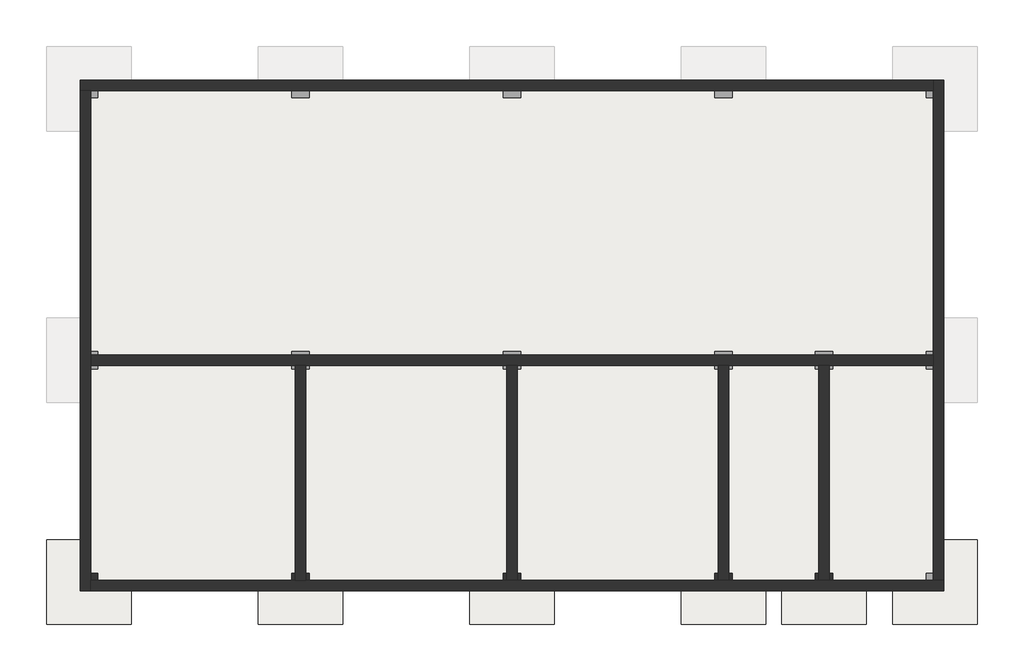
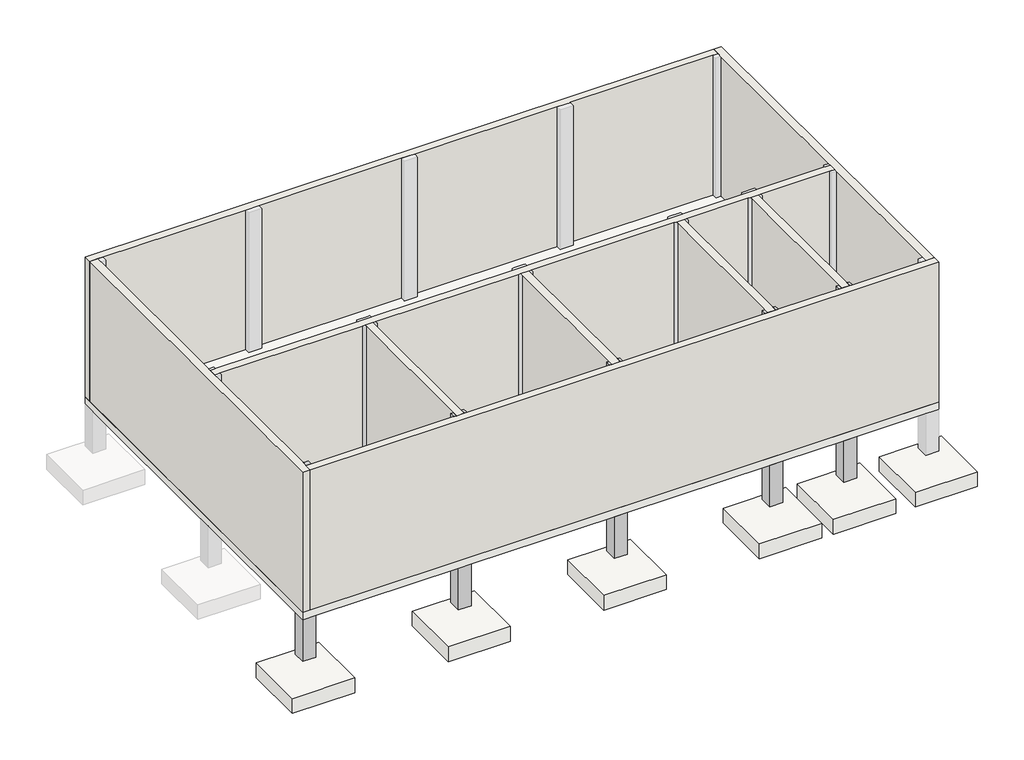
# One storey, part 1 of 2: 10 columns, 9 walls, 7 slabs.
"""IFC4 building model written with IfcOpenShell, lengths in millimetres."""

import ifcopenshell
import ifcopenshell.guid

model = None  # the IFC model being written
_history = None  # IfcOwnerHistory: only IFC2X3 demands one
_inside = {}  # id of a spatial element -> (the spatial element, [elements in it])
_under = {}  # id of a project, library or spatial element -> (it, [spatial elements below it])
_declared = {}  # id of a project -> (the project, [libraries it declares])
_typed = {}  # id of a type object -> (the type object, [elements of that type])
_made_of = {}  # id of a material, layer set ... -> (it, [elements and type objects made of it])


def new_model(schema):
    """Start an empty IFC model of exactly this schema.

    Asked for "IFC4X3", IfcOpenShell would pick the latest addendum, in which some entities
    have other attributes; the version numbers below select the first issue.
    IFC2X3 requires an IfcOwnerHistory on every rooted entity: one is made here for all.
    """
    global model, _history
    if schema == "IFC4X3":
        model = ifcopenshell.file(schema_version=(4, 3, 0, 0))
    else:
        model = ifcopenshell.file(schema=schema)
    _inside.clear()
    _under.clear()
    _declared.clear()
    _typed.clear()
    _made_of.clear()
    _history = None
    if model.schema == "IFC2X3":
        org = make("IfcOrganization", Name="unknown")
        user = make(
            "IfcPersonAndOrganization",
            ThePerson=make("IfcPerson", FamilyName="unknown"),
            TheOrganization=org,
        )
        app = make(
            "IfcApplication",
            ApplicationDeveloper=org,
            Version="unknown",
            ApplicationFullName="unknown",
            ApplicationIdentifier="unknown",
        )
        _history = make(
            "IfcOwnerHistory",
            OwningUser=user,
            OwningApplication=app,
            ChangeAction="ADDED",
            CreationDate=0,
        )
    return model


def make(cls, **values):
    """One entity of the class cls with the attributes given. An attribute that is None is left unset."""
    return model.create_entity(
        cls, **{name: value for name, value in values.items() if value is not None}
    )


def rooted(cls, **values):
    """An entity with a GlobalId (a new one), such as an element, a storey or a relation."""
    return make(cls, GlobalId=ifcopenshell.guid.new(), OwnerHistory=_history, **values)


def si_unit(unit_type, name, prefix=None):
    """IfcSIUnit, for example si_unit("LENGTHUNIT", "METRE", prefix="MILLI")."""
    return make("IfcSIUnit", UnitType=unit_type, Prefix=prefix, Name=name)


def assignment(units):
    """IfcUnitAssignment: the units of a project."""
    return None if units is None else make("IfcUnitAssignment", Units=units)


def point(xyz):
    """IfcCartesianPoint."""
    return None if xyz is None else make("IfcCartesianPoint", Coordinates=xyz)


def direction(xyz):
    """IfcDirection."""
    return None if xyz is None else make("IfcDirection", DirectionRatios=xyz)


def frame(location, z_axis=None, x_axis=None):
    """IfcAxis2Placement3D, a coordinate frame: its origin and axes. An axis left out is left unset."""
    return make(
        "IfcAxis2Placement3D",
        Location=point(location),
        Axis=direction(z_axis),
        RefDirection=direction(x_axis),
    )


def origin():
    """The frame at (0, 0, 0) with its axes left unset."""
    return frame((0.0, 0.0, 0.0))


def place(relative_to, where):
    """IfcLocalPlacement: puts the frame where relative to a parent placement (None: the world)."""
    return make(
        "IfcLocalPlacement", PlacementRelTo=relative_to, RelativePlacement=where
    )


def context(
    kind, dimensions, precision=None, world=None, true_north=None, identifier=None
):
    """IfcGeometricRepresentationContext, for example the 3D "Model" context."""
    return make(
        "IfcGeometricRepresentationContext",
        ContextIdentifier=identifier,
        ContextType=kind,
        CoordinateSpaceDimension=dimensions,
        Precision=precision,
        WorldCoordinateSystem=world,
        TrueNorth=true_north,
    )


def project(units=None, contexts=None):
    """IfcProject with its units and contexts."""
    return rooted(
        "IfcProject",
        Name="project",
        RepresentationContexts=contexts,
        UnitsInContext=assignment(units),
    )


def spatial(cls, under=None, at=None, **own):
    """A site, building, storey or space (cls), placed at a placement, below another one or the project."""
    s = rooted(cls, ObjectPlacement=at, **own)
    if under is not None:
        _under.setdefault(under.id(), (under, []))[1].append(s)
    return s


def polyline(points):
    """IfcPolyline through the points."""
    return make("IfcPolyline", Points=[point(p) for p in points])


def outline(outer, holes=None, kind="AREA"):
    """IfcArbitraryClosedProfileDef: a profile drawn as a closed curve; with holes, ...WithVoids."""
    if holes is None:
        return make("IfcArbitraryClosedProfileDef", ProfileType=kind, OuterCurve=outer)
    return make(
        "IfcArbitraryProfileDefWithVoids",
        ProfileType=kind,
        OuterCurve=outer,
        InnerCurves=holes,
    )


def extrude(swept, where, along, depth):
    """IfcExtrudedAreaSolid: the profile swept, set in the frame where, extruded along a direction by depth."""
    return make(
        "IfcExtrudedAreaSolid",
        SweptArea=swept,
        Position=where,
        ExtrudedDirection=direction(along),
        Depth=depth,
    )


def faces_of(points, faces, orient=None, outer=None):
    """IfcFace entities. A face is a list of loops; a loop is a list of indices into points, from 0.

    orient and outer hold one flag for each loop. By default every Orientation is true, the
    first loop of a face is its IfcFaceOuterBound and the others are IfcFaceBound.
    """
    made = []
    for i, loops in enumerate(faces):
        bounds = []
        for j, loop in enumerate(loops):
            is_outer = j == 0 if outer is None else outer[i][j]
            bounds.append(
                make(
                    "IfcFaceOuterBound" if is_outer else "IfcFaceBound",
                    Bound=make("IfcPolyLoop", Polygon=[points[k] for k in loop]),
                    Orientation=True if orient is None else orient[i][j],
                )
            )
        made.append(make("IfcFace", Bounds=bounds))
    return made


def faceted_brep(points, faces, orient=None, outer=None, voids=None):
    """IfcFacetedBrep: a solid bounded by flat faces; with voids (closed shells), ...WithVoids."""
    shared = [point(p) for p in points]
    hull = make("IfcClosedShell", CfsFaces=faces_of(shared, faces, orient, outer))
    if voids is None:
        return make("IfcFacetedBrep", Outer=hull)
    return make(
        "IfcFacetedBrepWithVoids",
        Outer=hull,
        Voids=[
            make(cls, CfsFaces=faces_of(shared, fs, o, b)) for cls, fs, o, b in voids
        ],
    )


def shape(context_of_items, identifier, shape_type, items):
    """IfcShapeRepresentation: the items that make up one representation, for example the "Body"."""
    return make(
        "IfcShapeRepresentation",
        ContextOfItems=context_of_items,
        RepresentationIdentifier=identifier,
        RepresentationType=shape_type,
        Items=items,
    )


def source(mapping_origin, context_of_items, identifier, shape_type, items):
    """IfcRepresentationMap: a shape defined once, which mapped items show again and again."""
    return make(
        "IfcRepresentationMap",
        MappingOrigin=mapping_origin,
        MappedRepresentation=shape(context_of_items, identifier, shape_type, items),
    )


def transform(
    local_origin,
    x_axis=None,
    y_axis=None,
    z_axis=None,
    scale=None,
    scale2=None,
    scale3=None,
    uniform=True,
):
    """IfcCartesianTransformationOperator3D, or its non-uniform kind. x_axis, y_axis, z_axis: its Axis1, 2, 3."""
    if uniform:
        return make(
            "IfcCartesianTransformationOperator3D",
            Axis1=direction(x_axis),
            Axis2=direction(y_axis),
            LocalOrigin=point(local_origin),
            Scale=scale,
            Axis3=direction(z_axis),
        )
    return make(
        "IfcCartesianTransformationOperator3DnonUniform",
        Axis1=direction(x_axis),
        Axis2=direction(y_axis),
        LocalOrigin=point(local_origin),
        Scale=scale,
        Axis3=direction(z_axis),
        Scale2=scale2,
        Scale3=scale3,
    )


def mapped(mapping_source, mapping_target):
    """IfcMappedItem: shows the shape of a source again, moved by a transform."""
    return make(
        "IfcMappedItem", MappingSource=mapping_source, MappingTarget=mapping_target
    )


def made_of(thing, what):
    """Note that an element or type object is made of a material, layer set ...; save() writes the relation."""
    if what is not None:
        _made_of.setdefault(what.id(), (what, []))[1].append(thing)
    return thing


def element(
    cls,
    number,
    at=None,
    inside=None,
    cuts=None,
    type_object=None,
    material=None,
    context=None,
    identifier="Body",
    shape_type=None,
    held_by="IfcProductDefinitionShape",
    body=None,
    shapes=None,
    **own,
):
    """One element of the class cls, such as IfcWall. Its Tag is "e" and its number.

    at: its placement. inside: the storey or other place that contains it. cuts: it is an
    opening in that element (IfcRelVoidsElement). A single representation is given by context,
    identifier, shape_type and body (its items); several are given by shapes. held_by: the class
    of the entity that holds the representations. save() writes the other relations.
    """
    e = rooted(cls, Tag="e%d" % number, ObjectPlacement=at, **own)
    if body is not None:
        shapes = [shape(context, identifier, shape_type, body)]
    if shapes is not None:
        e.Representation = make(held_by, Representations=shapes)
    if inside is not None:
        _inside.setdefault(inside.id(), (inside, []))[1].append(e)
    if cuts is not None:
        rooted(
            "IfcRelVoidsElement", RelatingBuildingElement=cuts, RelatedOpeningElement=e
        )
    if type_object is not None:
        _typed.setdefault(type_object.id(), (type_object, []))[1].append(e)
    return made_of(e, material)


def aggregate(whole, parts):
    """IfcRelAggregates: a whole, such as a stair, and the parts it consists of."""
    return rooted("IfcRelAggregates", RelatingObject=whole, RelatedObjects=parts)


def save(model, path):
    """Write the relations noted so far, then the file.

    IfcRelAggregates (storeys below a building ...), IfcRelContainedInSpatialStructure (elements
    in a storey), IfcRelDefinesByType, IfcRelAssociatesMaterial and IfcRelDeclares: one each for
    every whole, place, type object, material and project.
    """
    for whole, parts in _under.values():
        aggregate(whole, parts)
    for where, things in _inside.values():
        rooted(
            "IfcRelContainedInSpatialStructure",
            RelatedElements=things,
            RelatingStructure=where,
        )
    for kind, things in _typed.values():
        rooted("IfcRelDefinesByType", RelatedObjects=things, RelatingType=kind)
    for what, things in _made_of.values():
        rooted("IfcRelAssociatesMaterial", RelatedObjects=things, RelatingMaterial=what)
    for by, libraries in _declared.values():
        rooted("IfcRelDeclares", RelatingContext=by, RelatedDefinitions=libraries)
    model.write(path)


def foundation_rectangular_non_pile_2400_x_2400_x_600mm_9fdc1d6b(model_context):
    return source(origin(), model_context, "Body", "SweptSolid", [
        extrude(outline(polyline([(1200.0, 1200.0), (1200.0, -1200.0), (-1200.0, -1200.0), (-1200.0, 1200.0), (1200.0, 1200.0)])), frame((0.0, 0.0, -600.0), z_axis=(0.0, 0.0, 1.0), x_axis=(1.0, 0.0, 0.0)), (0.0, 0.0, 1.0), 600.0),
    ])


model = new_model("IFC4")

# Units and contexts
model_context = context("Model", 3, world=origin())
ifc_project = project(units=[si_unit("LENGTHUNIT", "METRE", prefix="MILLI")], contexts=[model_context])

# Site, building, storey
site = spatial("IfcSite", under=ifc_project)
building = spatial("IfcBuilding", under=site)
storey = spatial("IfcBuildingStorey", under=building, Name="1st FL GL+200", Elevation=0.0)

# Columns
placement = place(None, origin())
element("IfcColumn", 1, ObjectType="RC_Column_Rectangular : 500 x 500mm", at=placement, inside=storey, context=model_context, shape_type="SweptSolid", body=[
    extrude(outline(polyline([(-18445.7273237, -4314.0236875), (-18445.7273237, -4814.0236875), (-18945.7273237, -4814.0236875), (-18945.7273237, -4314.0236875), (-18445.7273237, -4314.0236875)])), frame((0.0, 0.0, -2000.0), z_axis=(0.0, 0.0, 1.0), x_axis=(1.0, 0.0, 0.0)), (0.0, 0.0, 1.0), 1700.0),
])
element("IfcColumn", 2, ObjectType="RC_Column_Rectangular : 500 x 500mm", at=placement, inside=storey, context=model_context, shape_type="SweptSolid", body=[
    extrude(outline(polyline([(-12445.7273237, -4314.0236875), (-12445.7273237, -4814.0236875), (-12945.7273237, -4814.0236875), (-12945.7273237, -4314.0236875), (-12445.7273237, -4314.0236875)])), frame((0.0, 0.0, -2000.0), z_axis=(0.0, 0.0, 1.0), x_axis=(1.0, 0.0, 0.0)), (0.0, 0.0, 1.0), 1700.0),
])
element("IfcColumn", 3, ObjectType="RC_Column_Rectangular : 500 x 500mm", at=placement, inside=storey, context=model_context, shape_type="SweptSolid", body=[
    extrude(outline(polyline([(-6445.7273237, -4314.0236875), (-6445.7273237, -4814.0236875), (-6945.7273237, -4814.0236875), (-6945.7273237, -4314.0236875), (-6445.7273237, -4314.0236875)])), frame((0.0, 0.0, -2000.0), z_axis=(0.0, 0.0, 1.0), x_axis=(1.0, 0.0, 0.0)), (0.0, 0.0, 1.0), 1700.0),
])
element("IfcColumn", 4, ObjectType="RC_Column_Rectangular : 500 x 500mm", at=placement, inside=storey, context=model_context, shape_type="SweptSolid", body=[
    extrude(outline(polyline([(-445.7273237, -4314.0236875), (-445.7273237, -4814.0236875), (-945.7273237, -4814.0236875), (-945.7273237, -4314.0236875), (-445.7273237, -4314.0236875)])), frame((0.0, 0.0, -2000.0), z_axis=(0.0, 0.0, 1.0), x_axis=(1.0, 0.0, 0.0)), (0.0, 0.0, 1.0), 1700.0),
])
element("IfcColumn", 5, ObjectType="RC_Column_Rectangular : 500 x 500mm", at=placement, inside=storey, context=model_context, shape_type="SweptSolid", body=[
    extrude(outline(polyline([(2404.2726763, -4314.0236875), (2404.2726763, -4814.0236875), (1904.2726763, -4814.0236875), (1904.2726763, -4314.0236875), (2404.2726763, -4314.0236875)])), frame((0.0, 0.0, -2000.0), z_axis=(0.0, 0.0, 1.0), x_axis=(1.0, 0.0, 0.0)), (0.0, 0.0, 1.0), 1700.0),
])
element("IfcColumn", 6, ObjectType="RC_Column_Rectangular : 500 x 500mm", at=placement, inside=storey, context=model_context, shape_type="Brep", body=[
    faceted_brep([(-18645.7273237, -4314.0236875, 0.0), (-18445.7273237, -4314.0236875, 0.0), (-18445.7273237, -4514.0236875, 0.0), (-18645.7273237, -4514.0236875, 0.0), (-18445.7273237, -4314.0236875, 5700.0), (-18645.7273237, -4314.0236875, 5300.0), (-18645.7273237, -4314.0236875, 5700.0), (-18595.7273237, -4314.0236875, 5700.0), (-18445.7273237, -4514.0236875, 5700.0), (-18645.7273237, -4514.0236875, 5700.0)], [[[0, 1, 2, 3]], [[4, 1, 0, 5, 6, 7]], [[1, 4, 8, 2]], [[4, 7, 6, 9, 8]], [[6, 5, 0, 3, 9]], [[3, 2, 8, 9]]]),
])
element("IfcColumn", 7, ObjectType="RC_Column_Rectangular : 500 x 500mm", at=placement, inside=storey, context=model_context, shape_type="Brep", body=[
    faceted_brep([(-12945.7273237, -4514.0236875, 0.0), (-12945.7273237, -4314.0236875, 0.0), (-12845.7273237, -4314.0236875, 0.0), (-12845.7273237, -4514.0236875, 0.0), (-12945.7273237, -4314.0236875, 5700.0), (-12945.7273237, -4514.0236875, 5300.0), (-12945.7273237, -4514.0236875, 5700.0), (-12945.7273237, -4464.0236875, 5700.0), (-12845.7273237, -4314.0236875, 5300.0), (-12845.7273237, -4314.0236875, 5700.0), (-12845.7273237, -4514.0236875, 5700.0), (-12870.7273237, -4314.0236875, 5700.0)], [[[0, 1, 2, 3]], [[4, 1, 0, 5, 6, 7]], [[3, 2, 8, 9, 10]], [[1, 4, 11, 9, 8, 2]], [[4, 7, 6, 10, 9, 11]], [[6, 5, 0, 3, 10]]]),
    faceted_brep([(-12445.7273237, -4314.0236875, 5700.0), (-12445.7273237, -4314.0236875, 0.0), (-12545.7273237, -4314.0236875, 0.0), (-12545.7273237, -4314.0236875, 5300.0), (-12545.7273237, -4314.0236875, 5700.0), (-12520.7273237, -4314.0236875, 5700.0), (-12445.7273237, -4464.0236875, 5700.0), (-12445.7273237, -4514.0236875, 5700.0), (-12445.7273237, -4514.0236875, 5300.0), (-12445.7273237, -4514.0236875, 0.0), (-12545.7273237, -4514.0236875, 5700.0), (-12545.7273237, -4514.0236875, 0.0)], [[[0, 1, 2, 3, 4, 5]], [[1, 0, 6, 7, 8, 9]], [[7, 6, 0, 5, 4, 10]], [[9, 8, 7, 10, 11]], [[2, 11, 10, 4, 3]], [[1, 9, 11, 2]]]),
])
element("IfcColumn", 8, ObjectType="RC_Column_Rectangular : 500 x 500mm", at=placement, inside=storey, context=model_context, shape_type="Brep", body=[
    faceted_brep([(-6945.7273237, -4514.0236875, 0.0), (-6945.7273237, -4314.0236875, 0.0), (-6845.7273237, -4314.0236875, 0.0), (-6845.7273237, -4514.0236875, 0.0), (-6945.7273237, -4314.0236875, 5700.0), (-6945.7273237, -4514.0236875, 5300.0), (-6945.7273237, -4514.0236875, 5700.0), (-6945.7273237, -4464.0236875, 5700.0), (-6845.7273237, -4314.0236875, 5300.0), (-6845.7273237, -4314.0236875, 5700.0), (-6845.7273237, -4514.0236875, 5700.0), (-6870.7273237, -4314.0236875, 5700.0)], [[[0, 1, 2, 3]], [[4, 1, 0, 5, 6, 7]], [[3, 2, 8, 9, 10]], [[1, 4, 11, 9, 8, 2]], [[4, 7, 6, 10, 9, 11]], [[6, 5, 0, 3, 10]]]),
    faceted_brep([(-6445.7273237, -4314.0236875, 5700.0), (-6445.7273237, -4314.0236875, 0.0), (-6545.7273237, -4314.0236875, 0.0), (-6545.7273237, -4314.0236875, 5300.0), (-6545.7273237, -4314.0236875, 5700.0), (-6520.7273237, -4314.0236875, 5700.0), (-6445.7273237, -4464.0236875, 5700.0), (-6445.7273237, -4514.0236875, 5700.0), (-6445.7273237, -4514.0236875, 5300.0), (-6445.7273237, -4514.0236875, 0.0), (-6545.7273237, -4514.0236875, 5700.0), (-6545.7273237, -4514.0236875, 0.0)], [[[0, 1, 2, 3, 4, 5]], [[1, 0, 6, 7, 8, 9]], [[7, 6, 0, 5, 4, 10]], [[9, 8, 7, 10, 11]], [[2, 11, 10, 4, 3]], [[1, 9, 11, 2]]]),
])
element("IfcColumn", 9, ObjectType="RC_Column_Rectangular : 500 x 500mm", at=placement, inside=storey, context=model_context, shape_type="Brep", body=[
    faceted_brep([(-945.7273237, -4514.0236875, 0.0), (-945.7273237, -4314.0236875, 0.0), (-845.7273237, -4314.0236875, 0.0), (-845.7273237, -4514.0236875, 0.0), (-945.7273237, -4314.0236875, 5700.0), (-945.7273237, -4514.0236875, 5300.0), (-945.7273237, -4514.0236875, 5700.0), (-945.7273237, -4464.0236875, 5700.0), (-845.7273237, -4314.0236875, 5300.0), (-845.7273237, -4314.0236875, 5700.0), (-845.7273237, -4514.0236875, 5700.0), (-870.7273237, -4314.0236875, 5700.0)], [[[0, 1, 2, 3]], [[4, 1, 0, 5, 6, 7]], [[3, 2, 8, 9, 10]], [[1, 4, 11, 9, 8, 2]], [[4, 7, 6, 10, 9, 11]], [[6, 5, 0, 3, 10]]]),
    faceted_brep([(-445.7273237, -4314.0236875, 5700.0), (-445.7273237, -4314.0236875, 0.0), (-545.7273237, -4314.0236875, 0.0), (-545.7273237, -4314.0236875, 5300.0), (-545.7273237, -4314.0236875, 5700.0), (-520.7273237, -4314.0236875, 5700.0), (-445.7273237, -4464.0236875, 5700.0), (-445.7273237, -4514.0236875, 5700.0), (-445.7273237, -4514.0236875, 5300.0), (-445.7273237, -4514.0236875, 0.0), (-545.7273237, -4514.0236875, 5700.0), (-545.7273237, -4514.0236875, 0.0)], [[[0, 1, 2, 3, 4, 5]], [[1, 0, 6, 7, 8, 9]], [[7, 6, 0, 5, 4, 10]], [[9, 8, 7, 10, 11]], [[2, 11, 10, 4, 3]], [[1, 9, 11, 2]]]),
])
element("IfcColumn", 10, ObjectType="RC_Column_Rectangular : 500 x 500mm", at=placement, inside=storey, context=model_context, shape_type="Brep", body=[
    faceted_brep([(1904.2726763, -4514.0236875, 0.0), (1904.2726763, -4314.0236875, 0.0), (2004.2726763, -4314.0236875, 0.0), (2004.2726763, -4514.0236875, 0.0), (1904.2726763, -4314.0236875, 5700.0), (1904.2726763, -4514.0236875, 5300.0), (1904.2726763, -4514.0236875, 5700.0), (1904.2726763, -4464.0236875, 5700.0), (2004.2726763, -4314.0236875, 5300.0), (2004.2726763, -4314.0236875, 5700.0), (2004.2726763, -4514.0236875, 5700.0), (1979.2726763, -4314.0236875, 5700.0)], [[[0, 1, 2, 3]], [[4, 1, 0, 5, 6, 7]], [[3, 2, 8, 9, 10]], [[1, 4, 11, 9, 8, 2]], [[4, 7, 6, 10, 9, 11]], [[6, 5, 0, 3, 10]]]),
    faceted_brep([(2404.2726763, -4314.0236875, 5700.0), (2404.2726763, -4314.0236875, 0.0), (2304.2726763, -4314.0236875, 0.0), (2304.2726763, -4314.0236875, 5300.0), (2304.2726763, -4314.0236875, 5700.0), (2329.2726763, -4314.0236875, 5700.0), (2404.2726763, -4464.0236875, 5700.0), (2404.2726763, -4514.0236875, 5700.0), (2404.2726763, -4514.0236875, 5300.0), (2404.2726763, -4514.0236875, 0.0), (2304.2726763, -4514.0236875, 5700.0), (2304.2726763, -4514.0236875, 0.0)], [[[0, 1, 2, 3, 4, 5]], [[1, 0, 6, 7, 8, 9]], [[7, 6, 0, 5, 4, 10]], [[9, 8, 7, 10, 11]], [[2, 11, 10, 4, 3]], [[1, 9, 11, 2]]]),
])

# Slabs
element("IfcSlab", 11, ObjectType="H_FL_ACS_RC Slab_T150", at=placement, inside=storey, context=model_context, shape_type="Brep", body=[
    faceted_brep([(5554.2726763, -4814.0236875, -300.0), (5054.2726763, -4814.0236875, -300.0), (2404.2726763, -4814.0236875, -300.0), (1904.2726763, -4814.0236875, -300.0), (-445.7273237, -4814.0236875, -300.0), (-945.7273237, -4814.0236875, -300.0), (-6445.7273237, -4814.0236875, -300.0), (-6945.7273237, -4814.0236875, -300.0), (-12445.7273237, -4814.0236875, -300.0), (-12945.7273237, -4814.0236875, -300.0), (-18445.7273237, -4814.0236875, -300.0), (-18945.7273237, -4814.0236875, -300.0), (-18945.7273237, -4314.0236875, -300.0), (-18945.7273237, 1485.9763125, -300.0), (-18945.7273237, 1985.9763125, -300.0), (-18945.7273237, 9185.9763125, -300.0), (-18945.7273237, 9685.9763125, -300.0), (-18445.7273237, 9685.9763125, -300.0), (-12945.7273237, 9685.9763125, -300.0), (-12445.7273237, 9685.9763125, -300.0), (-6945.7273237, 9685.9763125, -300.0), (-6445.7273237, 9685.9763125, -300.0), (-945.7273237, 9685.9763125, -300.0), (-445.7273237, 9685.9763125, -300.0), (5054.2726763, 9685.9763125, -300.0), (5554.2726763, 9685.9763125, -300.0), (5554.2726763, 9185.9763125, -300.0), (5554.2726763, 1985.9763125, -300.0), (5554.2726763, 1485.9763125, -300.0), (5554.2726763, -4314.0236875, -300.0), (5554.2726763, -4814.0236875, 0.0), (5554.2726763, 9685.9763125, 0.0), (-18945.7273237, 9685.9763125, 0.0), (-18945.7273237, -4814.0236875, 0.0)], [[[0, 1, 2, 3, 4, 5, 6, 7, 8, 9, 10, 11, 12, 13, 14, 15, 16, 17, 18, 19, 20, 21, 22, 23, 24, 25, 26, 27, 28, 29]], [[30, 31, 32, 33]], [[11, 10, 9, 8, 7, 6, 5, 4, 3, 2, 1, 0, 30, 33]], [[16, 15, 14, 13, 12, 11, 33, 32]], [[25, 24, 23, 22, 21, 20, 19, 18, 17, 16, 32, 31]], [[0, 29, 28, 27, 26, 25, 31, 30]]]),
])
foundation_rectangular_non_pile_2400_x_2400_x_600mm_shape = foundation_rectangular_non_pile_2400_x_2400_x_600mm_9fdc1d6b(model_context)
element("IfcSlab", 12, ObjectType="Foundation Rectangular(Non-Pile) : 2400 x 2400 x 600mm", at=placement, inside=storey, context=model_context, shape_type="MappedRepresentation", body=[
    mapped(foundation_rectangular_non_pile_2400_x_2400_x_600mm_shape, transform((-18695.7273237, -4564.0236875, -2600.0), x_axis=(1.0, 0.0, 0.0), y_axis=(0.0, 1.0, 0.0), z_axis=(0.0, 0.0, 1.0))),
])
element("IfcSlab", 13, ObjectType="Foundation Rectangular(Non-Pile) : 2400 x 2400 x 600mm", at=placement, inside=storey, context=model_context, shape_type="MappedRepresentation", body=[
    mapped(foundation_rectangular_non_pile_2400_x_2400_x_600mm_shape, transform((-12695.7273237, -4564.0236875, -2600.0), x_axis=(1.0, 0.0, 0.0), y_axis=(0.0, 1.0, 0.0), z_axis=(0.0, 0.0, 1.0))),
])
element("IfcSlab", 14, ObjectType="Foundation Rectangular(Non-Pile) : 2400 x 2400 x 600mm", at=placement, inside=storey, context=model_context, shape_type="MappedRepresentation", body=[
    mapped(foundation_rectangular_non_pile_2400_x_2400_x_600mm_shape, transform((-6695.7273237, -4564.0236875, -2600.0), x_axis=(1.0, 0.0, 0.0), y_axis=(0.0, 1.0, 0.0), z_axis=(0.0, 0.0, 1.0))),
])
element("IfcSlab", 15, ObjectType="Foundation Rectangular(Non-Pile) : 2400 x 2400 x 600mm", at=placement, inside=storey, context=model_context, shape_type="MappedRepresentation", body=[
    mapped(foundation_rectangular_non_pile_2400_x_2400_x_600mm_shape, transform((-695.7273237, -4564.0236875, -2600.0), x_axis=(1.0, 0.0, 0.0), y_axis=(0.0, 1.0, 0.0), z_axis=(0.0, 0.0, 1.0))),
])
element("IfcSlab", 16, ObjectType="Foundation Rectangular(Non-Pile) : 2400 x 2400 x 600mm", at=placement, inside=storey, context=model_context, shape_type="MappedRepresentation", body=[
    mapped(foundation_rectangular_non_pile_2400_x_2400_x_600mm_shape, transform((5304.2726763, -4564.0236875, -2600.0), x_axis=(1.0, 0.0, 0.0), y_axis=(0.0, 1.0, 0.0), z_axis=(0.0, 0.0, 1.0))),
])
element("IfcSlab", 17, ObjectType="Foundation Rectangular(Non-Pile) : 2400 x 2400 x 600mm", at=placement, inside=storey, context=model_context, shape_type="MappedRepresentation", body=[
    mapped(foundation_rectangular_non_pile_2400_x_2400_x_600mm_shape, transform((2154.2726763, -4564.0236875, -2600.0), x_axis=(1.0, 0.0, 0.0), y_axis=(0.0, 1.0, 0.0), z_axis=(0.0, 0.0, 1.0))),
])

# Walls
element("IfcWall", 18, ObjectType="일반 - 300mm", at=placement, inside=storey, context=model_context, shape_type="Brep", body=[
    faceted_brep([(-18945.7273237, 9385.9763125, 0.0), (-18645.7273237, 9385.9763125, 0.0), (-18445.7273237, 9385.9763125, 0.0), (-12945.7273237, 9385.9763125, 0.0), (-12445.7273237, 9385.9763125, 0.0), (-6945.7273237, 9385.9763125, 0.0), (-6445.7273237, 9385.9763125, 0.0), (-945.7273237, 9385.9763125, 0.0), (-445.7273237, 9385.9763125, 0.0), (5054.2726763, 9385.9763125, 0.0), (5254.2726763, 9385.9763125, 0.0), (5254.2726763, 9385.9763125, 5300.0), (5254.2726763, 9385.9763125, 5700.0), (5054.2726763, 9385.9763125, 5700.0), (-433.0273237, 9385.9763125, 5700.0), (-445.7273237, 9385.9763125, 5700.0), (-945.7273237, 9385.9763125, 5700.0), (-6445.7273237, 9385.9763125, 5700.0), (-6945.7273237, 9385.9763125, 5700.0), (-12445.7273237, 9385.9763125, 5700.0), (-12945.7273237, 9385.9763125, 5700.0), (-18445.7273237, 9385.9763125, 5700.0), (-18645.7273237, 9385.9763125, 5700.0), (-18945.7273237, 9385.9763125, 5700.0), (5254.2726763, 9685.9763125, 0.0), (-18945.7273237, 9685.9763125, 0.0), (-18945.7273237, 9685.9763125, 5700.0), (5254.2726763, 9685.9763125, 5700.0)], [[[0, 1, 2, 3, 4, 5, 6, 7, 8, 9, 10, 11, 12, 13, 14, 15, 16, 17, 18, 19, 20, 21, 22, 23]], [[24, 25, 26, 27]], [[10, 9, 8, 7, 6, 5, 4, 3, 2, 1, 0, 25, 24]], [[25, 0, 23, 26]], [[10, 24, 27, 12, 11]], [[23, 22, 21, 20, 19, 18, 17, 16, 15, 14, 13, 12, 27, 26]]]),
])
element("IfcWall", 19, ObjectType="일반 - 300mm", at=placement, inside=storey, context=model_context, shape_type="Brep", body=[
    faceted_brep([(-18645.7273237, -4814.0236875, 0.0), (-18645.7273237, -4514.0236875, 0.0), (-18645.7273237, -4314.0236875, 0.0), (-18645.7273237, 1485.9763125, 0.0), (-18645.7273237, 1585.9763125, 0.0), (-18645.7273237, 1885.9763125, 0.0), (-18645.7273237, 1985.9763125, 0.0), (-18645.7273237, 9185.9763125, 0.0), (-18645.7273237, 9385.9763125, 0.0), (-18645.7273237, 9385.9763125, 5700.0), (-18645.7273237, 9185.9763125, 5700.0), (-18645.7273237, 1985.9763125, 5700.0), (-18645.7273237, 1885.9763125, 5700.0), (-18645.7273237, 1585.9763125, 5700.0), (-18645.7273237, 1485.9763125, 5700.0), (-18645.7273237, -4314.0236875, 5700.0), (-18645.7273237, -4514.0236875, 5700.0), (-18645.7273237, -4814.0236875, 5700.0), (-18945.7273237, 9385.9763125, 0.0), (-18945.7273237, -4814.0236875, 0.0), (-18945.7273237, -4814.0236875, 5700.0), (-18945.7273237, 9385.9763125, 5700.0)], [[[0, 1, 2, 3, 4, 5, 6, 7, 8, 9, 10, 11, 12, 13, 14, 15, 16, 17]], [[18, 19, 20, 21]], [[8, 7, 6, 5, 4, 3, 2, 1, 0, 19, 18]], [[19, 0, 17, 20]], [[8, 18, 21, 9]], [[17, 16, 15, 14, 13, 12, 11, 10, 9, 21, 20]]]),
])
element("IfcWall", 20, ObjectType="일반 - 300mm", at=placement, inside=storey, context=model_context, shape_type="Brep", body=[
    faceted_brep([(5554.2726763, -4514.0236875, 0.0), (5254.2726763, -4514.0236875, 0.0), (5054.2726763, -4514.0236875, 0.0), (2404.2726763, -4514.0236875, 0.0), (2304.2726763, -4514.0236875, 0.0), (2004.2726763, -4514.0236875, 0.0), (1904.2726763, -4514.0236875, 0.0), (-445.7273237, -4514.0236875, 0.0), (-545.7273237, -4514.0236875, 0.0), (-845.7273237, -4514.0236875, 0.0), (-945.7273237, -4514.0236875, 0.0), (-6445.7273237, -4514.0236875, 0.0), (-6545.7273237, -4514.0236875, 0.0), (-6845.7273237, -4514.0236875, 0.0), (-6945.7273237, -4514.0236875, 0.0), (-12445.7273237, -4514.0236875, 0.0), (-12545.7273237, -4514.0236875, 0.0), (-12845.7273237, -4514.0236875, 0.0), (-12945.7273237, -4514.0236875, 0.0), (-18445.7273237, -4514.0236875, 0.0), (-18645.7273237, -4514.0236875, 0.0), (-18645.7273237, -4514.0236875, 5300.0), (-18645.7273237, -4514.0236875, 5700.0), (-18445.7273237, -4514.0236875, 5700.0), (-12945.7273237, -4514.0236875, 5700.0), (-12845.7273237, -4514.0236875, 5700.0), (-12545.7273237, -4514.0236875, 5700.0), (-12445.7273237, -4514.0236875, 5700.0), (-6945.7273237, -4514.0236875, 5700.0), (-6845.7273237, -4514.0236875, 5700.0), (-6545.7273237, -4514.0236875, 5700.0), (-6445.7273237, -4514.0236875, 5700.0), (-945.7273237, -4514.0236875, 5700.0), (-845.7273237, -4514.0236875, 5700.0), (-545.7273237, -4514.0236875, 5700.0), (-445.7273237, -4514.0236875, 5700.0), (1904.2726763, -4514.0236875, 5700.0), (2004.2726763, -4514.0236875, 5700.0), (2304.2726763, -4514.0236875, 5700.0), (2404.2726763, -4514.0236875, 5700.0), (5054.2726763, -4514.0236875, 5700.0), (5254.2726763, -4514.0236875, 5700.0), (5554.2726763, -4514.0236875, 5700.0), (-18645.7273237, -4814.0236875, 0.0), (5554.2726763, -4814.0236875, 0.0), (5554.2726763, -4814.0236875, 5700.0), (-18645.7273237, -4814.0236875, 5700.0)], [[[0, 1, 2, 3, 4, 5, 6, 7, 8, 9, 10, 11, 12, 13, 14, 15, 16, 17, 18, 19, 20, 21, 22, 23, 24, 25, 26, 27, 28, 29, 30, 31, 32, 33, 34, 35, 36, 37, 38, 39, 40, 41, 42]], [[43, 44, 45, 46]], [[20, 19, 18, 17, 16, 15, 14, 13, 12, 11, 10, 9, 8, 7, 6, 5, 4, 3, 2, 1, 0, 44, 43]], [[44, 0, 42, 45]], [[20, 43, 46, 22, 21]], [[42, 41, 40, 39, 38, 37, 36, 35, 34, 33, 32, 31, 30, 29, 28, 27, 26, 25, 24, 23, 22, 46, 45]]]),
])
element("IfcWall", 21, ObjectType="일반 - 300mm", at=placement, inside=storey, context=model_context, shape_type="Brep", body=[
    faceted_brep([(5254.2726763, 9685.9763125, 0.0), (5254.2726763, 9385.9763125, 0.0), (5254.2726763, 9185.9763125, 0.0), (5254.2726763, 1985.9763125, 0.0), (5254.2726763, 1885.9763125, 0.0), (5254.2726763, 1585.9763125, 0.0), (5254.2726763, 1485.9763125, 0.0), (5254.2726763, -4314.0236875, 0.0), (5254.2726763, -4514.0236875, 0.0), (5254.2726763, -4514.0236875, 5700.0), (5254.2726763, -4314.0236875, 5700.0), (5254.2726763, 1485.9763125, 5700.0), (5254.2726763, 1585.9763125, 5700.0), (5254.2726763, 1885.9763125, 5700.0), (5254.2726763, 1985.9763125, 5700.0), (5254.2726763, 9185.9763125, 5700.0), (5254.2726763, 9385.9763125, 5700.0), (5254.2726763, 9685.9763125, 5700.0), (5554.2726763, -4514.0236875, 0.0), (5554.2726763, 9685.9763125, 0.0), (5554.2726763, 9685.9763125, 5700.0), (5554.2726763, -4514.0236875, 5700.0)], [[[0, 1, 2, 3, 4, 5, 6, 7, 8, 9, 10, 11, 12, 13, 14, 15, 16, 17]], [[18, 19, 20, 21]], [[8, 7, 6, 5, 4, 3, 2, 1, 0, 19, 18]], [[19, 0, 17, 20]], [[8, 18, 21, 9]], [[17, 16, 15, 14, 13, 12, 11, 10, 9, 21, 20]]]),
])
element("IfcWall", 22, ObjectType="일반 - 300mm", at=placement, inside=storey, context=model_context, shape_type="Brep", body=[
    faceted_brep([(-18645.7273237, 1585.9763125, 0.0), (-18445.7273237, 1585.9763125, 0.0), (-12945.7273237, 1585.9763125, 0.0), (-12845.7273237, 1585.9763125, 0.0), (-12545.7273237, 1585.9763125, 0.0), (-12445.7273237, 1585.9763125, 0.0), (-6945.7273237, 1585.9763125, 0.0), (-6845.7273237, 1585.9763125, 0.0), (-6545.7273237, 1585.9763125, 0.0), (-6445.7273237, 1585.9763125, 0.0), (-945.7273237, 1585.9763125, 0.0), (-845.7273237, 1585.9763125, 0.0), (-545.7273237, 1585.9763125, 0.0), (-445.7273237, 1585.9763125, 0.0), (1904.2726763, 1585.9763125, 0.0), (2004.2726763, 1585.9763125, 0.0), (2304.2726763, 1585.9763125, 0.0), (2404.2726763, 1585.9763125, 0.0), (5054.2726763, 1585.9763125, 0.0), (5254.2726763, 1585.9763125, 0.0), (5254.2726763, 1585.9763125, 5700.0), (5054.2726763, 1585.9763125, 5700.0), (2404.2726763, 1585.9763125, 5700.0), (2304.2726763, 1585.9763125, 5700.0), (2004.2726763, 1585.9763125, 5700.0), (1904.2726763, 1585.9763125, 5700.0), (-445.7273237, 1585.9763125, 5700.0), (-545.7273237, 1585.9763125, 5700.0), (-845.7273237, 1585.9763125, 5700.0), (-945.7273237, 1585.9763125, 5700.0), (-6445.7273237, 1585.9763125, 5700.0), (-6545.7273237, 1585.9763125, 5700.0), (-6845.7273237, 1585.9763125, 5700.0), (-6945.7273237, 1585.9763125, 5700.0), (-12445.7273237, 1585.9763125, 5700.0), (-12545.7273237, 1585.9763125, 5700.0), (-12845.7273237, 1585.9763125, 5700.0), (-12945.7273237, 1585.9763125, 5700.0), (-18445.7273237, 1585.9763125, 5700.0), (-18645.7273237, 1585.9763125, 5700.0), (5254.2726763, 1885.9763125, 0.0), (5054.2726763, 1885.9763125, 0.0), (2404.2726763, 1885.9763125, 0.0), (1904.2726763, 1885.9763125, 0.0), (-445.7273237, 1885.9763125, 0.0), (-945.7273237, 1885.9763125, 0.0), (-6445.7273237, 1885.9763125, 0.0), (-6945.7273237, 1885.9763125, 0.0), (-12445.7273237, 1885.9763125, 0.0), (-12945.7273237, 1885.9763125, 0.0), (-18445.7273237, 1885.9763125, 0.0), (-18645.7273237, 1885.9763125, 0.0), (-18645.7273237, 1885.9763125, 5700.0), (-18445.7273237, 1885.9763125, 5700.0), (-12945.7273237, 1885.9763125, 5700.0), (-12445.7273237, 1885.9763125, 5700.0), (-6945.7273237, 1885.9763125, 5700.0), (-6445.7273237, 1885.9763125, 5700.0), (-945.7273237, 1885.9763125, 5700.0), (-445.7273237, 1885.9763125, 5700.0), (1904.2726763, 1885.9763125, 5700.0), (2404.2726763, 1885.9763125, 5700.0), (5054.2726763, 1885.9763125, 5700.0), (5254.2726763, 1885.9763125, 5700.0)], [[[0, 1, 2, 3, 4, 5, 6, 7, 8, 9, 10, 11, 12, 13, 14, 15, 16, 17, 18, 19, 20, 21, 22, 23, 24, 25, 26, 27, 28, 29, 30, 31, 32, 33, 34, 35, 36, 37, 38, 39]], [[40, 41, 42, 43, 44, 45, 46, 47, 48, 49, 50, 51, 52, 53, 54, 55, 56, 57, 58, 59, 60, 61, 62, 63]], [[19, 18, 17, 16, 15, 14, 13, 12, 11, 10, 9, 8, 7, 6, 5, 4, 3, 2, 1, 0, 51, 50, 49, 48, 47, 46, 45, 44, 43, 42, 41, 40]], [[19, 40, 63, 20]], [[51, 0, 39, 52]], [[39, 38, 37, 36, 35, 34, 33, 32, 31, 30, 29, 28, 27, 26, 25, 24, 23, 22, 21, 20, 63, 62, 61, 60, 59, 58, 57, 56, 55, 54, 53, 52]]]),
])
element("IfcWall", 23, ObjectType="일반 - 300mm", at=placement, inside=storey, context=model_context, shape_type="Brep", body=[
    faceted_brep([(2004.2726763, 1585.9763125, 0.0), (2004.2726763, 1485.9763125, 0.0), (2004.2726763, -4314.0236875, 0.0), (2004.2726763, -4514.0236875, 0.0), (2004.2726763, -4514.0236875, 5700.0), (2004.2726763, -4314.0236875, 5700.0), (2004.2726763, 1485.9763125, 5700.0), (2004.2726763, 1585.9763125, 5700.0), (2304.2726763, -4514.0236875, 0.0), (2304.2726763, -4314.0236875, 0.0), (2304.2726763, 1485.9763125, 0.0), (2304.2726763, 1585.9763125, 0.0), (2304.2726763, 1585.9763125, 5700.0), (2304.2726763, 1485.9763125, 5700.0), (2304.2726763, -4314.0236875, 5700.0), (2304.2726763, -4514.0236875, 5700.0)], [[[0, 1, 2, 3, 4, 5, 6, 7]], [[8, 9, 10, 11, 12, 13, 14, 15]], [[3, 2, 1, 0, 11, 10, 9, 8]], [[3, 8, 15, 4]], [[11, 0, 7, 12]], [[7, 6, 5, 4, 15, 14, 13, 12]]]),
])
element("IfcWall", 24, ObjectType="일반 - 300mm", at=placement, inside=storey, context=model_context, shape_type="Brep", body=[
    faceted_brep([(-845.7273237, 1585.9763125, 0.0), (-845.7273237, 1485.9763125, 0.0), (-845.7273237, -4314.0236875, 0.0), (-845.7273237, -4514.0236875, 0.0), (-845.7273237, -4514.0236875, 5700.0), (-845.7273237, -4314.0236875, 5700.0), (-845.7273237, 1485.9763125, 5700.0), (-845.7273237, 1585.9763125, 5700.0), (-545.7273237, -4514.0236875, 0.0), (-545.7273237, -4314.0236875, 0.0), (-545.7273237, 1485.9763125, 0.0), (-545.7273237, 1585.9763125, 0.0), (-545.7273237, 1585.9763125, 5700.0), (-545.7273237, 1485.9763125, 5700.0), (-545.7273237, -4314.0236875, 5700.0), (-545.7273237, -4514.0236875, 5700.0)], [[[0, 1, 2, 3, 4, 5, 6, 7]], [[8, 9, 10, 11, 12, 13, 14, 15]], [[3, 2, 1, 0, 11, 10, 9, 8]], [[3, 8, 15, 4]], [[11, 0, 7, 12]], [[7, 6, 5, 4, 15, 14, 13, 12]]]),
])
element("IfcWall", 25, ObjectType="일반 - 300mm", at=placement, inside=storey, context=model_context, shape_type="Brep", body=[
    faceted_brep([(-6845.7273237, 1585.9763125, 0.0), (-6845.7273237, 1485.9763125, 0.0), (-6845.7273237, -4314.0236875, 0.0), (-6845.7273237, -4514.0236875, 0.0), (-6845.7273237, -4514.0236875, 5700.0), (-6845.7273237, -4314.0236875, 5700.0), (-6845.7273237, 1485.9763125, 5700.0), (-6845.7273237, 1585.9763125, 5700.0), (-6545.7273237, -4514.0236875, 0.0), (-6545.7273237, -4314.0236875, 0.0), (-6545.7273237, 1485.9763125, 0.0), (-6545.7273237, 1585.9763125, 0.0), (-6545.7273237, 1585.9763125, 5700.0), (-6545.7273237, 1485.9763125, 5700.0), (-6545.7273237, -4314.0236875, 5700.0), (-6545.7273237, -4514.0236875, 5700.0)], [[[0, 1, 2, 3, 4, 5, 6, 7]], [[8, 9, 10, 11, 12, 13, 14, 15]], [[3, 2, 1, 0, 11, 10, 9, 8]], [[3, 8, 15, 4]], [[11, 0, 7, 12]], [[7, 6, 5, 4, 15, 14, 13, 12]]]),
])
element("IfcWall", 26, ObjectType="일반 - 300mm", at=placement, inside=storey, context=model_context, shape_type="Brep", body=[
    faceted_brep([(-12845.7273237, 1585.9763125, 0.0), (-12845.7273237, 1485.9763125, 0.0), (-12845.7273237, -4314.0236875, 0.0), (-12845.7273237, -4514.0236875, 0.0), (-12845.7273237, -4514.0236875, 5700.0), (-12845.7273237, -4314.0236875, 5700.0), (-12845.7273237, 1485.9763125, 5700.0), (-12845.7273237, 1585.9763125, 5700.0), (-12545.7273237, -4514.0236875, 0.0), (-12545.7273237, -4314.0236875, 0.0), (-12545.7273237, 1485.9763125, 0.0), (-12545.7273237, 1585.9763125, 0.0), (-12545.7273237, 1585.9763125, 5700.0), (-12545.7273237, 1485.9763125, 5700.0), (-12545.7273237, -4314.0236875, 5700.0), (-12545.7273237, -4514.0236875, 5700.0)], [[[0, 1, 2, 3, 4, 5, 6, 7]], [[8, 9, 10, 11, 12, 13, 14, 15]], [[3, 2, 1, 0, 11, 10, 9, 8]], [[3, 8, 15, 4]], [[11, 0, 7, 12]], [[7, 6, 5, 4, 15, 14, 13, 12]]]),
])

save(model, "model.ifc")

# Revit data of these elements
# Project information
#   프로젝트 발행 날짜 = "발행 날짜"
#   프로젝트 상태 = "프로젝트 상태"
#   클라이언트 이름 = "소유자"
#   프로젝트 주소 = "주소를 여기에 입력"
#   프로젝트 이름 = "프로젝트 이름"
#   프로젝트 번호 = "0001"
# Grids (mm)
#   "Y16": line (2154.273, 3257.871) -> (2154.273, -8233.19)
#   "X2": line (-12695.727, -8233.19) -> (-12695.727, 14438.726)
#   "X3": line (-6695.727, -8233.19) -> (-6695.727, 14438.726)
#   "X4": line (-695.727, -8233.19) -> (-695.727, 14438.726)
#   "X5": line (5304.273, -8233.19) -> (5304.273, 14438.726)
#   "Y2": line (9794.388, 1735.976) -> (-24604.07, 1735.976)
#   "Y1": line (9794.388, -4564.024) -> (-24604.07, -4564.024)
#   "Y3": line (9794.388, 9435.976) -> (-24604.07, 9435.976)
#   "X1": line (-18695.727, -8233.19) -> (-18695.727, 14438.726)
# Type "RC_Column_Rectangular : 500 x 500mm"
#   b = 500 mm
#   h = 500 mm
#   Structural Material [instance default] = 콘크리트, 현장타설 회색
# Type "H_FL_ACS_RC Slab_T150"
#   Function = 0
#   Layers, outside or top first: 300 mm no material (function 1)
# Type "Foundation Rectangular(Non-Pile) : 2400 x 2400 x 600mm"
#   Width = 2400 mm
#   Length = 2400 mm
#   Foundation Thickness = 600 mm
#   Structural Material [instance default] = 콘크리트 - 현장타설 콘크리트
#   Assembly Code = ""
# Type "일반 - 300mm"
#   Layers, outside or top first: 300 mm no material (function 1)
# Elements 1, 2, 3, 4, 5, 6, 7, 8, 9, 10 (IfcColumn, "RC_Column_Rectangular : 500 x 500mm")
#   Structural Material = 콘크리트, 현장타설 회색
#   Phase Created = 신축
#   Materials on its faces: "콘크리트, 현장타설 회색"
# Element 11 (IfcSlab, "H_FL_ACS_RC Slab_T150")
#   Height Offset From Level = 0 mm
#   Phase Created = 신축
#   Materials on its faces: "기본 바닥"
# Elements 12, 13, 14, 15, 16, 17 (IfcSlab, "Foundation Rectangular(Non-Pile) : 2400 x 2400 x 600mm")
#   Structural Material = 콘크리트 - 현장타설 콘크리트
#   Phase Created = 신축
#   Materials on its faces: "콘크리트 - 현장타설 콘크리트"
# Elements 18, 19, 20, 21, 22, 23, 24, 25, 26 (IfcWall, "일반 - 300mm")
#   Comments = ""
#   Top Offset = 0 mm
#   Base Offset = 0 mm
#   wall height = 6000 mm
#   Phase Created = 신축
#   Base Constraint = 1st FL GL+200
#   Top Constraint = 2nd FL GL+6,200
#   Materials on its faces: "기본 벽"
# Materials
#   "콘크리트, 현장타설 회색": class "콘크리트", colour RGB 192 192 192, transparency 0, Description = "현장타설 콘크리트", Cost = 0
#   "콘크리트 - 현장타설 콘크리트": class "콘크리트", colour RGB 192 192 192, transparency 0, Cost = 0
#   "기본 바닥": class "다양한", colour RGB 127 127 127, transparency 0, Cost = 0
#   "기본 벽": class "다양한", colour RGB 128 128 128, transparency 0, Cost = 0
# Room at (-6795.727, 5585.976) mm, phase "신축", upper level "1st FL GL+200", upper offset 6000 mm, lower offset 0 mm
#   Base Finish = "B01"
#   Ceiling Finish = "C95A"
#   Wall Finish = "W01B"
#   Floor Finish = "F03"
#   Number = "1101"
#   Name = "test"
#   Wall Base Material = "Masonry Wall"
#   Wall Finish 1 = "Plastering"
#   Wall Finish 2 = "Acrylic Emulsion Paint"
#   Wall Finish Remark = "THK 12 Plaster"
#   Floor Base Material = "Concrete Slab"
#   Floor Finish 1 = "Steel Trowel Finish"
#   Floor Finish 2 = "Acid Resistant Paint"
#   Base Base Material = "Concrete Wall"
#   Base Finish 1 = "Acrylic Emulsion Paint"
#   Base Finish Remark = "H=100"
#   Ceiling Base Material = "Concrete Slab"
#   Ceiling Finish 1 = "Acoustic Tiled Ceiling System (T-Bar)"
#   Ceiling Finish Remark = "600x600, CH=3000"
#   H_Room W = 0 mm
#   H_Room L = 0 mm
#   H_Room H or CH = 0 mm
#   Wall Finish Style = Acrylic Emulsion Paint on Cement Plaster
#   Floor Finish Style = Acid Resistant Paint on Steel Trowel Finish
#   Base Finish Style = Acrylic Emulsion Paint
#   Ceiling Finish Style = Suspended Acoustic Tiled Ceiling (T-Bar)
# Room at (3729.273, -1414.024) mm, phase "신축", upper level "1st FL GL+200", upper offset 6000 mm, lower offset 0 mm
#   Base Finish = "B03"
#   Ceiling Finish = "C95A"
#   Wall Finish = "W01B"
#   Floor Finish = "F06A"
#   Number = "1102"
#   Name = "test"
#   H_Room W = 0 mm
#   H_Room L = 0 mm
#   H_Room H or CH = 0 mm
# Room at (729.273, -1414.024) mm, phase "신축", upper level "1st FL GL+200", upper offset 6000 mm, lower offset 0 mm
#   Base Finish = "B32"
#   Ceiling Finish = "C96A"
#   Wall Finish = "W04B"
#   Floor Finish = "F31B"
#   Number = "1103"
#   Name = "test"
#   H_Room W = 0 mm
#   H_Room L = 0 mm
#   H_Room H or CH = 0 mm
# Room at (-3695.727, -1414.024) mm, phase "신축", upper level "1st FL GL+200", upper offset 6000 mm, lower offset 0 mm
#   Base Finish = "B33"
#   Ceiling Finish = "C01"
#   Wall Finish = "W32D"
#   Floor Finish = "F34A"
#   Number = "1104"
#   Name = "test"
#   H_Room W = 0 mm
#   H_Room L = 0 mm
#   H_Room H or CH = 0 mm
# Room at (-15695.727, -1414.024) mm, phase "신축", upper level "1st FL GL+200", upper offset 6000 mm, lower offset 0 mm
#   Base Finish = "B01"
#   Ceiling Finish = "C96A"
#   Wall Finish = "W01B"
#   Floor Finish = "F41"
#   Number = "1106"
#   Name = "test"
#   H_Room W = 0 mm
#   H_Room L = 0 mm
#   H_Room H or CH = 0 mm
# Room at (-9695.727, -1414.024) mm, phase "신축", upper level "1st FL GL+200", upper offset 6000 mm, lower offset 0 mm
#   Base Finish = "B35A"
#   Ceiling Finish = "C95A"
#   Wall Finish = "W01A"
#   Floor Finish = "F34B"
#   Number = "1105"
#   Name = "test"
#   H_Room W = 0 mm
#   H_Room L = 0 mm
#   H_Room H or CH = 0 mm
